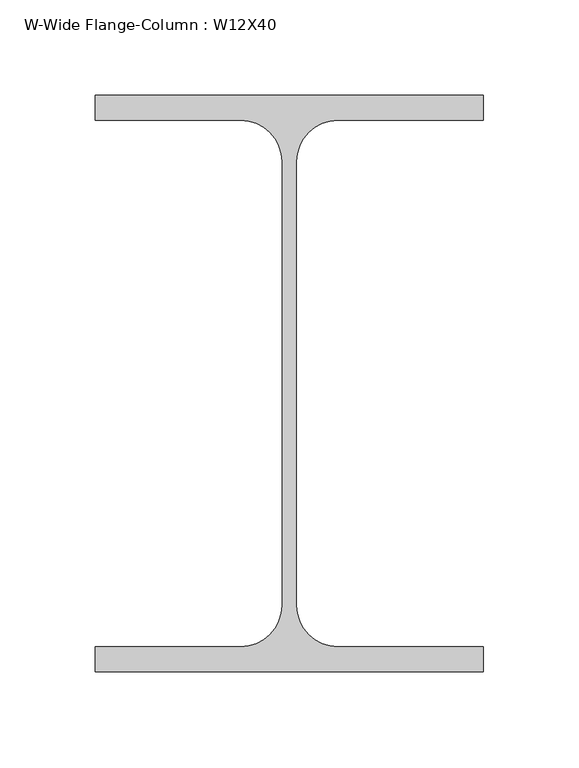
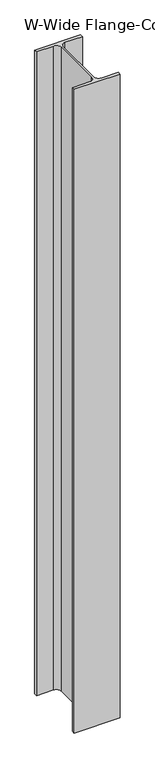
"""IFC4 building model written with IfcOpenShell, lengths in millimetres: column geometry, W-Wide Flange-Column : W12X40."""

from ifc_helpers import new_model, si_unit, point, frame, frame_2d, origin, place, context, project, spatial, polyline, circle_curve, trimmed, segment, composite_curve, outline, extrude, source, transform, mapped, element, save


def w_wide_flange_column_w12x40_bec10e2f(model_context):
    return source(origin(), model_context, "Body", "SweptSolid", [
        extrude(outline(composite_curve([segment(polyline([(101.727, 151.13), (101.727, 138.049), (25.5905, 138.049)]), True, "CONTINUOUS"), segment(trimmed(circle_curve(frame_2d((25.5905, 116.205)), 21.844), [point((25.5905, 138.049))], [point((3.7465, 116.205))], True, "CARTESIAN"), True, "CONTINUOUS"), segment(polyline([(3.7465, 116.205), (3.7465, -116.205)]), True, "CONTINUOUS"), segment(trimmed(circle_curve(frame_2d((25.5905, -116.205)), 21.844), [point((3.7465, -116.205))], [point((25.5905, -138.049))], True, "CARTESIAN"), True, "CONTINUOUS"), segment(polyline([(25.5905, -138.049), (101.727, -138.049), (101.727, -151.13), (-101.727, -151.13), (-101.727, -138.049), (-25.5905, -138.049)]), True, "CONTINUOUS"), segment(trimmed(circle_curve(frame_2d((-25.5905, -116.205)), 21.844), [point((-25.5905, -138.049))], [point((-3.7465, -116.205))], True, "CARTESIAN"), True, "CONTINUOUS"), segment(polyline([(-3.7465, -116.205), (-3.7465, 116.205)]), True, "CONTINUOUS"), segment(trimmed(circle_curve(frame_2d((-25.5905, 116.205)), 21.844), [point((-3.7465, 116.205))], [point((-25.5905, 138.049))], True, "CARTESIAN"), True, "CONTINUOUS"), segment(polyline([(-25.5905, 138.049), (-101.727, 138.049), (-101.727, 151.13), (101.727, 151.13)]), True, "CONTINUOUS")], self_intersect=False)), frame((0.0, 0.0, 29006.8), z_axis=(0.0, 0.0, 1.0), x_axis=(1.0, 0.0, 0.0)), (0.0, 0.0, 1.0), 3010.5945312),
    ])


if __name__ == "__main__":
    model = new_model("IFC4")
    model_context = context("Model", 3, world=origin())
    ifc_project = project(units=[si_unit("LENGTHUNIT", "METRE", prefix="MILLI")], contexts=[model_context])
    site = spatial("IfcSite", under=ifc_project)
    building = spatial("IfcBuilding", under=site)
    placement = place(None, origin())
    w_wide_flange_column_w12x40_shape = w_wide_flange_column_w12x40_bec10e2f(model_context)
    element("IfcColumn", 1, ObjectType="W-Wide Flange-Column : W12X40", at=placement, inside=building, context=model_context, shape_type="MappedRepresentation", body=[
        mapped(w_wide_flange_column_w12x40_shape, transform((0.0, 0.0, 0.0), x_axis=(1.0, 0.0, 0.0), y_axis=(0.0, 1.0, 0.0), z_axis=(0.0, 0.0, 1.0))),
    ])
    save(model, "model.ifc")

# Revit data of these elements
# Type "W-Wide Flange-Column : W12X40"
#   Assembly Code = "B10"
#   W = 40
#   bf = 0' - 8.01"
#   d = 0' - 11.9"
#   k = 0' - 1 3/8"
#   kr = 0' - 0.86"
#   tf = 0' - 0.515"
#   tw = 0' - 0.295"
#   A = 0.08125 SF
#   Structural Material [instance default] = Steel ASTM A992
# Element 1 (IfcColumn, "W-Wide Flange-Column : W12X40")
#   Materials on its faces: "Steel ASTM A992"
# Materials
#   "Steel ASTM A992": class "Metal", colour RGB 199 199 199, transparency 0, Description = "Structural steel 50ksi", Cost = 0
